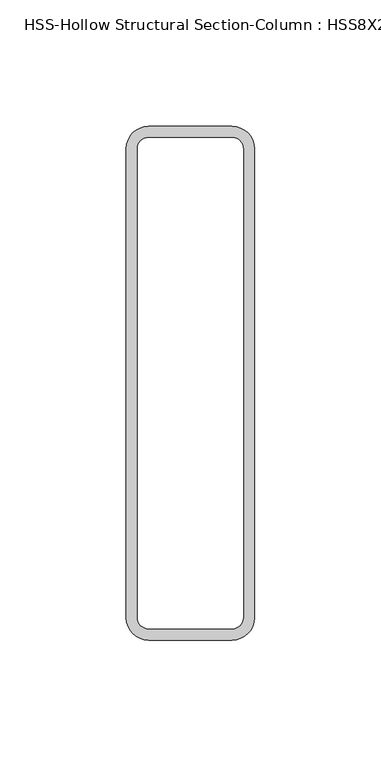
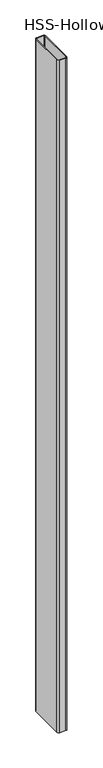
"""IFC4 building model written with IfcOpenShell, lengths in millimetres: column geometry, HSS-Hollow Structural Section-Column : HSS8X2X3/16."""

import ifcopenshell
import ifcopenshell.guid

model = None  # the IFC model being written
_history = None  # IfcOwnerHistory: only IFC2X3 demands one
_inside = {}  # id of a spatial element -> (the spatial element, [elements in it])
_under = {}  # id of a project, library or spatial element -> (it, [spatial elements below it])
_declared = {}  # id of a project -> (the project, [libraries it declares])
_typed = {}  # id of a type object -> (the type object, [elements of that type])
_made_of = {}  # id of a material, layer set ... -> (it, [elements and type objects made of it])


def new_model(schema):
    """Start an empty IFC model of exactly this schema.

    Asked for "IFC4X3", IfcOpenShell would pick the latest addendum, in which some entities
    have other attributes; the version numbers below select the first issue.
    IFC2X3 requires an IfcOwnerHistory on every rooted entity: one is made here for all.
    """
    global model, _history
    if schema == "IFC4X3":
        model = ifcopenshell.file(schema_version=(4, 3, 0, 0))
    else:
        model = ifcopenshell.file(schema=schema)
    _inside.clear()
    _under.clear()
    _declared.clear()
    _typed.clear()
    _made_of.clear()
    _history = None
    if model.schema == "IFC2X3":
        org = make("IfcOrganization", Name="unknown")
        user = make(
            "IfcPersonAndOrganization",
            ThePerson=make("IfcPerson", FamilyName="unknown"),
            TheOrganization=org,
        )
        app = make(
            "IfcApplication",
            ApplicationDeveloper=org,
            Version="unknown",
            ApplicationFullName="unknown",
            ApplicationIdentifier="unknown",
        )
        _history = make(
            "IfcOwnerHistory",
            OwningUser=user,
            OwningApplication=app,
            ChangeAction="ADDED",
            CreationDate=0,
        )
    return model


def make(cls, **values):
    """One entity of the class cls with the attributes given. An attribute that is None is left unset."""
    return model.create_entity(
        cls, **{name: value for name, value in values.items() if value is not None}
    )


def rooted(cls, **values):
    """An entity with a GlobalId (a new one), such as an element, a storey or a relation."""
    return make(cls, GlobalId=ifcopenshell.guid.new(), OwnerHistory=_history, **values)


def si_unit(unit_type, name, prefix=None):
    """IfcSIUnit, for example si_unit("LENGTHUNIT", "METRE", prefix="MILLI")."""
    return make("IfcSIUnit", UnitType=unit_type, Prefix=prefix, Name=name)


def assignment(units):
    """IfcUnitAssignment: the units of a project."""
    return None if units is None else make("IfcUnitAssignment", Units=units)


def point(xyz):
    """IfcCartesianPoint."""
    return None if xyz is None else make("IfcCartesianPoint", Coordinates=xyz)


def direction(xyz):
    """IfcDirection."""
    return None if xyz is None else make("IfcDirection", DirectionRatios=xyz)


def frame(location, z_axis=None, x_axis=None):
    """IfcAxis2Placement3D, a coordinate frame: its origin and axes. An axis left out is left unset."""
    return make(
        "IfcAxis2Placement3D",
        Location=point(location),
        Axis=direction(z_axis),
        RefDirection=direction(x_axis),
    )


def frame_2d(location, x_axis=None):
    """IfcAxis2Placement2D, a coordinate frame in the plane: its origin and x axis."""
    return make(
        "IfcAxis2Placement2D", Location=point(location), RefDirection=direction(x_axis)
    )


def origin():
    """The frame at (0, 0, 0) with its axes left unset."""
    return frame((0.0, 0.0, 0.0))


def place(relative_to, where):
    """IfcLocalPlacement: puts the frame where relative to a parent placement (None: the world)."""
    return make(
        "IfcLocalPlacement", PlacementRelTo=relative_to, RelativePlacement=where
    )


def context(
    kind, dimensions, precision=None, world=None, true_north=None, identifier=None
):
    """IfcGeometricRepresentationContext, for example the 3D "Model" context."""
    return make(
        "IfcGeometricRepresentationContext",
        ContextIdentifier=identifier,
        ContextType=kind,
        CoordinateSpaceDimension=dimensions,
        Precision=precision,
        WorldCoordinateSystem=world,
        TrueNorth=true_north,
    )


def project(units=None, contexts=None):
    """IfcProject with its units and contexts."""
    return rooted(
        "IfcProject",
        Name="project",
        RepresentationContexts=contexts,
        UnitsInContext=assignment(units),
    )


def spatial(cls, under=None, at=None, **own):
    """A site, building, storey or space (cls), placed at a placement, below another one or the project."""
    s = rooted(cls, ObjectPlacement=at, **own)
    if under is not None:
        _under.setdefault(under.id(), (under, []))[1].append(s)
    return s


def polyline(points):
    """IfcPolyline through the points."""
    return make("IfcPolyline", Points=[point(p) for p in points])


def circle_curve(where, radius):
    """IfcCircle in the frame where."""
    return make("IfcCircle", Position=where, Radius=radius)


def trimmed(basis, trim1, trim2, sense, master):
    """IfcTrimmedCurve: the piece of a basis curve between two trims."""
    return make(
        "IfcTrimmedCurve",
        BasisCurve=basis,
        Trim1=trim1,
        Trim2=trim2,
        SenseAgreement=sense,
        MasterRepresentation=master,
    )


def segment(curve, same_sense, transition):
    """IfcCompositeCurveSegment."""
    return make(
        "IfcCompositeCurveSegment",
        Transition=transition,
        SameSense=same_sense,
        ParentCurve=curve,
    )


def composite_curve(segments, self_intersect=None):
    """IfcCompositeCurve: segments joined end to end."""
    return make("IfcCompositeCurve", Segments=segments, SelfIntersect=self_intersect)


def outline(outer, holes=None, kind="AREA"):
    """IfcArbitraryClosedProfileDef: a profile drawn as a closed curve; with holes, ...WithVoids."""
    if holes is None:
        return make("IfcArbitraryClosedProfileDef", ProfileType=kind, OuterCurve=outer)
    return make(
        "IfcArbitraryProfileDefWithVoids",
        ProfileType=kind,
        OuterCurve=outer,
        InnerCurves=holes,
    )


def extrude(swept, where, along, depth):
    """IfcExtrudedAreaSolid: the profile swept, set in the frame where, extruded along a direction by depth."""
    return make(
        "IfcExtrudedAreaSolid",
        SweptArea=swept,
        Position=where,
        ExtrudedDirection=direction(along),
        Depth=depth,
    )


def shape(context_of_items, identifier, shape_type, items):
    """IfcShapeRepresentation: the items that make up one representation, for example the "Body"."""
    return make(
        "IfcShapeRepresentation",
        ContextOfItems=context_of_items,
        RepresentationIdentifier=identifier,
        RepresentationType=shape_type,
        Items=items,
    )


def source(mapping_origin, context_of_items, identifier, shape_type, items):
    """IfcRepresentationMap: a shape defined once, which mapped items show again and again."""
    return make(
        "IfcRepresentationMap",
        MappingOrigin=mapping_origin,
        MappedRepresentation=shape(context_of_items, identifier, shape_type, items),
    )


def transform(
    local_origin,
    x_axis=None,
    y_axis=None,
    z_axis=None,
    scale=None,
    scale2=None,
    scale3=None,
    uniform=True,
):
    """IfcCartesianTransformationOperator3D, or its non-uniform kind. x_axis, y_axis, z_axis: its Axis1, 2, 3."""
    if uniform:
        return make(
            "IfcCartesianTransformationOperator3D",
            Axis1=direction(x_axis),
            Axis2=direction(y_axis),
            LocalOrigin=point(local_origin),
            Scale=scale,
            Axis3=direction(z_axis),
        )
    return make(
        "IfcCartesianTransformationOperator3DnonUniform",
        Axis1=direction(x_axis),
        Axis2=direction(y_axis),
        LocalOrigin=point(local_origin),
        Scale=scale,
        Axis3=direction(z_axis),
        Scale2=scale2,
        Scale3=scale3,
    )


def mapped(mapping_source, mapping_target):
    """IfcMappedItem: shows the shape of a source again, moved by a transform."""
    return make(
        "IfcMappedItem", MappingSource=mapping_source, MappingTarget=mapping_target
    )


def made_of(thing, what):
    """Note that an element or type object is made of a material, layer set ...; save() writes the relation."""
    if what is not None:
        _made_of.setdefault(what.id(), (what, []))[1].append(thing)
    return thing


def element(
    cls,
    number,
    at=None,
    inside=None,
    cuts=None,
    type_object=None,
    material=None,
    context=None,
    identifier="Body",
    shape_type=None,
    held_by="IfcProductDefinitionShape",
    body=None,
    shapes=None,
    **own,
):
    """One element of the class cls, such as IfcWall. Its Tag is "e" and its number.

    at: its placement. inside: the storey or other place that contains it. cuts: it is an
    opening in that element (IfcRelVoidsElement). A single representation is given by context,
    identifier, shape_type and body (its items); several are given by shapes. held_by: the class
    of the entity that holds the representations. save() writes the other relations.
    """
    e = rooted(cls, Tag="e%d" % number, ObjectPlacement=at, **own)
    if body is not None:
        shapes = [shape(context, identifier, shape_type, body)]
    if shapes is not None:
        e.Representation = make(held_by, Representations=shapes)
    if inside is not None:
        _inside.setdefault(inside.id(), (inside, []))[1].append(e)
    if cuts is not None:
        rooted(
            "IfcRelVoidsElement", RelatingBuildingElement=cuts, RelatedOpeningElement=e
        )
    if type_object is not None:
        _typed.setdefault(type_object.id(), (type_object, []))[1].append(e)
    return made_of(e, material)


def aggregate(whole, parts):
    """IfcRelAggregates: a whole, such as a stair, and the parts it consists of."""
    return rooted("IfcRelAggregates", RelatingObject=whole, RelatedObjects=parts)


def save(model, path):
    """Write the relations noted so far, then the file.

    IfcRelAggregates (storeys below a building ...), IfcRelContainedInSpatialStructure (elements
    in a storey), IfcRelDefinesByType, IfcRelAssociatesMaterial and IfcRelDeclares: one each for
    every whole, place, type object, material and project.
    """
    for whole, parts in _under.values():
        aggregate(whole, parts)
    for where, things in _inside.values():
        rooted(
            "IfcRelContainedInSpatialStructure",
            RelatedElements=things,
            RelatingStructure=where,
        )
    for kind, things in _typed.values():
        rooted("IfcRelDefinesByType", RelatedObjects=things, RelatingType=kind)
    for what, things in _made_of.values():
        rooted("IfcRelAssociatesMaterial", RelatedObjects=things, RelatingMaterial=what)
    for by, libraries in _declared.values():
        rooted("IfcRelDeclares", RelatingContext=by, RelatedDefinitions=libraries)
    model.write(path)


def hss_hollow_structural_section_column_hss8x2x3_16_47370f60(model_context):
    return source(origin(), model_context, "Body", "SweptSolid", [
        extrude(outline(composite_curve([segment(trimmed(circle_curve(frame_2d((16.5608, 92.7608)), 8.8392), [point((16.5608, 101.6))], [point((25.4, 92.7608))], False, "CARTESIAN"), True, "CONTINUOUS"), segment(polyline([(25.4, 92.7608), (25.4, -92.7608)]), True, "CONTINUOUS"), segment(trimmed(circle_curve(frame_2d((16.5608, -92.7608)), 8.8392), [point((25.4, -92.7608))], [point((16.5608, -101.6))], False, "CARTESIAN"), True, "CONTINUOUS"), segment(polyline([(16.5608, -101.6), (-16.5608, -101.6)]), True, "CONTINUOUS"), segment(trimmed(circle_curve(frame_2d((-16.5608, -92.7608)), 8.8392), [point((-16.5608, -101.6))], [point((-25.4, -92.7608))], False, "CARTESIAN"), True, "CONTINUOUS"), segment(polyline([(-25.4, -92.7608), (-25.4, 92.7608)]), True, "CONTINUOUS"), segment(trimmed(circle_curve(frame_2d((-16.5608, 92.7608)), 8.8392), [point((-25.4, 92.7608))], [point((-16.5608, 101.6))], False, "CARTESIAN"), True, "CONTINUOUS"), segment(polyline([(-16.5608, 101.6), (16.5608, 101.6)]), True, "CONTINUOUS")], self_intersect=False), holes=[composite_curve([segment(polyline([(16.5608, 97.1804), (-16.5608, 97.1804)]), True, "CONTINUOUS"), segment(trimmed(circle_curve(frame_2d((-16.5608, 92.7608)), 4.4196), [point((-16.5608, 97.1804))], [point((-20.9804, 92.7608))], True, "CARTESIAN"), True, "CONTINUOUS"), segment(polyline([(-20.9804, 92.7608), (-20.9804, -92.7608)]), True, "CONTINUOUS"), segment(trimmed(circle_curve(frame_2d((-16.5608, -92.7608)), 4.4196), [point((-20.9804, -92.7608))], [point((-16.5608, -97.1804))], True, "CARTESIAN"), True, "CONTINUOUS"), segment(polyline([(-16.5608, -97.1804), (16.5608, -97.1804)]), True, "CONTINUOUS"), segment(trimmed(circle_curve(frame_2d((16.5608, -92.7608)), 4.4196), [point((16.5608, -97.1804))], [point((20.9804, -92.7608))], True, "CARTESIAN"), True, "CONTINUOUS"), segment(polyline([(20.9804, -92.7608), (20.9804, 92.7608)]), True, "CONTINUOUS"), segment(trimmed(circle_curve(frame_2d((16.5608, 92.7608)), 4.4196), [point((20.9804, 92.7608))], [point((16.5608, 97.1804))], True, "CARTESIAN"), True, "CONTINUOUS")], self_intersect=False)]), frame((0.0, 0.0, -1200.0), z_axis=(0.0, 0.0, 1.0), x_axis=(1.0, 0.0, 0.0)), (0.0, 0.0, 1.0), 3644.0),
    ])


if __name__ == "__main__":
    model = new_model("IFC4")
    model_context = context("Model", 3, world=origin())
    ifc_project = project(units=[si_unit("LENGTHUNIT", "METRE", prefix="MILLI")], contexts=[model_context])
    site = spatial("IfcSite", under=ifc_project)
    building = spatial("IfcBuilding", under=site)
    placement = place(None, origin())
    hss_hollow_structural_section_column_hss8x2x3_16_shape = hss_hollow_structural_section_column_hss8x2x3_16_47370f60(model_context)
    element("IfcColumn", 1, ObjectType="HSS-Hollow Structural Section-Column : HSS8X2X3/16", at=placement, inside=building, context=model_context, shape_type="MappedRepresentation", body=[
        mapped(hss_hollow_structural_section_column_hss8x2x3_16_shape, transform((0.0, 0.0, 0.0), x_axis=(1.0, 0.0, 0.0), y_axis=(0.0, 1.0, 0.0), z_axis=(0.0, 0.0, 1.0))),
    ])
    save(model, "model.ifc")

# Revit data of these elements
# Project information
#   Project Issue Date = "Issue Date"
#   Project Status = "Project Status"
#   Client Name = "Owner"
#   Project Address = "Enter address here"
#   Project Name = "Project Name"
#   Project Number = "0001"
# Type "HSS-Hollow Structural Section-Column : HSS8X2X3/16"
#   Assembly Code = "B10"
#   Shape = "Rect."
#   Cost = 1
#   W = 12
#   Ht = 203.2 mm
#   b = 50.8 mm
#   kr = 8.839 mm
#   t = 4.42 mm
#   A = 0.00211612 m²
#   Structural Material [instance default] = Steel ASTM A500, Grade B, Rectangular and Square
# Element 1 (IfcColumn, "HSS-Hollow Structural Section-Column : HSS8X2X3/16")
#   Structural Material = Metal - Steel 43-275
#   Materials on its faces: "Metal - Steel 43-275"
# Materials
#   "Steel ASTM A500, Grade B, Rectangular and Square": class "Metal", colour RGB 199 199 199, transparency 0, Description = "Carbon steel", Cost = 0
#   "Metal - Steel 43-275": class "Metal", colour RGB 247 247 247, transparency 0, Cost = 0
